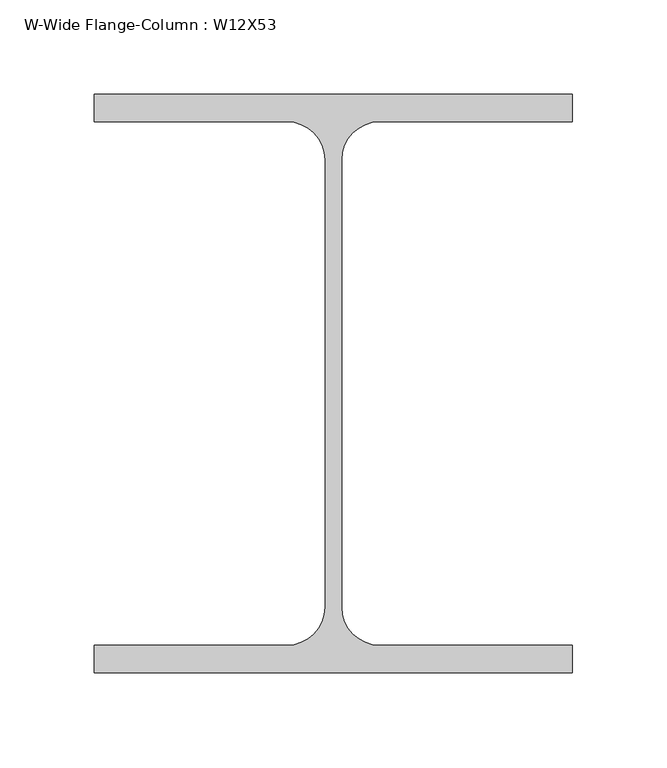
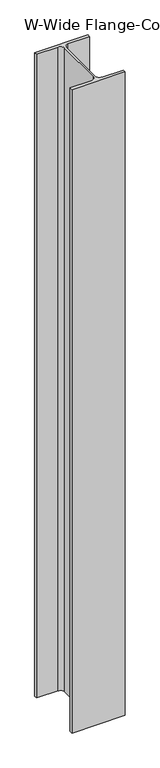
"""IFC4 building model written with IfcOpenShell, lengths in millimetres: column geometry, W-Wide Flange-Column : W12X53."""

from ifc_helpers import new_model, si_unit, point, frame, frame_2d, origin, place, context, project, spatial, polyline, circle_curve, trimmed, segment, composite_curve, outline, extrude, source, transform, mapped, element, save


def w_wide_flange_column_w12x53_e560d531(model_context):
    return source(origin(), model_context, "Body", "SweptSolid", [
        extrude(outline(composite_curve([segment(polyline([(127.0, 153.67), (127.0, 139.065), (24.7015, 139.065)]), True, "CONTINUOUS"), segment(trimmed(circle_curve(frame_2d((24.7015, 118.745)), 20.32), [point((24.7015, 139.065))], [point((4.3815, 118.745))], True, "CARTESIAN"), True, "CONTINUOUS"), segment(polyline([(4.3815, 118.745), (4.3815, -118.745)]), True, "CONTINUOUS"), segment(trimmed(circle_curve(frame_2d((24.7015, -118.745)), 20.32), [point((4.3815, -118.745))], [point((24.7015, -139.065))], True, "CARTESIAN"), True, "CONTINUOUS"), segment(polyline([(24.7015, -139.065), (127.0, -139.065), (127.0, -153.67), (-127.0, -153.67), (-127.0, -139.065), (-24.7015, -139.065)]), True, "CONTINUOUS"), segment(trimmed(circle_curve(frame_2d((-24.7015, -118.745)), 20.32), [point((-24.7015, -139.065))], [point((-4.3815, -118.745))], True, "CARTESIAN"), True, "CONTINUOUS"), segment(polyline([(-4.3815, -118.745), (-4.3815, 118.745)]), True, "CONTINUOUS"), segment(trimmed(circle_curve(frame_2d((-24.7015, 118.745)), 20.32), [point((-4.3815, 118.745))], [point((-24.7015, 139.065))], True, "CARTESIAN"), True, "CONTINUOUS"), segment(polyline([(-24.7015, 139.065), (-127.0, 139.065), (-127.0, 153.67), (127.0, 153.67)]), True, "CONTINUOUS")], self_intersect=False)), frame((0.0, 0.0, 9163.05), z_axis=(0.0, 0.0, 1.0), x_axis=(1.0, 0.0, 0.0)), (0.0, 0.0, 1.0), 3244.85),
    ])


if __name__ == "__main__":
    model = new_model("IFC4")
    model_context = context("Model", 3, world=origin())
    ifc_project = project(units=[si_unit("LENGTHUNIT", "METRE", prefix="MILLI")], contexts=[model_context])
    site = spatial("IfcSite", under=ifc_project)
    building = spatial("IfcBuilding", under=site)
    placement = place(None, origin())
    w_wide_flange_column_w12x53_shape = w_wide_flange_column_w12x53_e560d531(model_context)
    element("IfcColumn", 1, ObjectType="W-Wide Flange-Column : W12X53", at=placement, inside=building, context=model_context, shape_type="MappedRepresentation", body=[
        mapped(w_wide_flange_column_w12x53_shape, transform((0.0, 0.0, 0.0), x_axis=(1.0, 0.0, 0.0), y_axis=(0.0, 1.0, 0.0), z_axis=(0.0, 0.0, 1.0))),
    ])
    save(model, "model.ifc")

# Revit data of these elements
# Type "W-Wide Flange-Column : W12X53"
#   Assembly Code = "B10"
#   W = 53
#   bf = 0' - 10"
#   d = 1' - 0.1"
#   k = 0' - 1 3/8"
#   kr = 0' - 0.8"
#   tf = 0' - 0.575"
#   tw = 0' - 0.345"
#   A = 0.108333 SF
#   Structural Material [instance default] = Steel ASTM A992
# Element 1 (IfcColumn, "W-Wide Flange-Column : W12X53")
#   Materials on its faces: "Steel ASTM A992"
# Materials
#   "Steel ASTM A992": class "Metal", colour RGB 199 199 199, transparency 0, Description = "Structural steel 50ksi", Cost = 0
